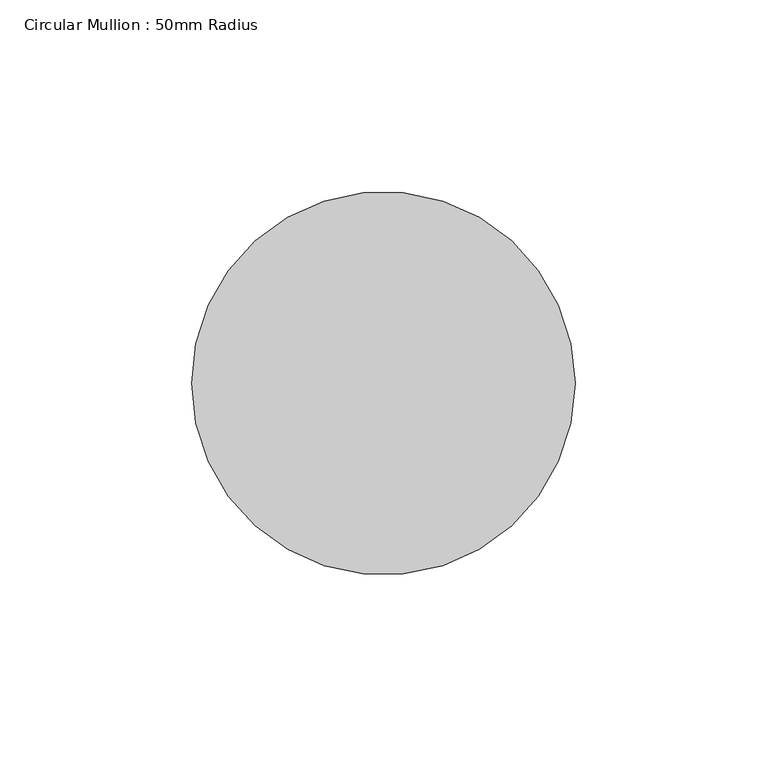
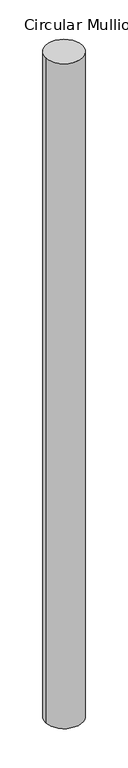
"""IFC4 building model written with IfcOpenShell, lengths in millimetres: member geometry, Circular Mullion : 50mm Radius."""

from ifc_helpers import new_model, si_unit, point, frame, origin, origin_2d, place, context, project, spatial, circle_curve, trimmed, segment, composite_curve, outline, extrude, source, transform, mapped, element, save


def circular_mullion_50mm_radius_83dc5a6d(model_context):
    return source(origin(), model_context, "Body", "SweptSolid", [
        extrude(outline(composite_curve([segment(trimmed(circle_curve(origin_2d(), 50.0), [point((50.0, 0.0))], [point((-50.0, 0.0))], False, "CARTESIAN"), True, "CONTINUOUS"), segment(trimmed(circle_curve(origin_2d(), 50.0), [point((-50.0, 0.0))], [point((50.0, 0.0))], False, "CARTESIAN"), True, "CONTINUOUS")], self_intersect=False)), frame((0.0, 0.0, -1906.709071), z_axis=(0.0, 0.0, 1.0), x_axis=(1.0, 0.0, 0.0)), (0.0, 0.0, 1.0), 1906.709071),
    ])


if __name__ == "__main__":
    model = new_model("IFC4")
    model_context = context("Model", 3, world=origin())
    ifc_project = project(units=[si_unit("LENGTHUNIT", "METRE", prefix="MILLI")], contexts=[model_context])
    site = spatial("IfcSite", under=ifc_project)
    building = spatial("IfcBuilding", under=site)
    placement = place(None, origin())
    circular_mullion_50mm_radius_shape = circular_mullion_50mm_radius_83dc5a6d(model_context)
    element("IfcMember", 1, ObjectType="Circular Mullion : 50mm Radius", at=placement, inside=building, context=model_context, shape_type="MappedRepresentation", body=[
        mapped(circular_mullion_50mm_radius_shape, transform((0.0, 0.0, 0.0), x_axis=(1.0, 0.0, 0.0), y_axis=(0.0, 1.0, 0.0), z_axis=(0.0, 0.0, 1.0))),
    ])
    save(model, "model.ifc")

# Revit data of these elements
# Type "Circular Mullion : 50mm Radius"
#   built-in parameter 1007350 = 0.164042 (stored number, unit not read)
# Element 1 (IfcMember, "Circular Mullion : 50mm Radius")
#   Materials on its faces: "Aluminium"
# Materials
#   "Aluminium": class "Metal", colour RGB 247 247 247, transparency 0, Description = "Aluminium 6061", Cost = 0
